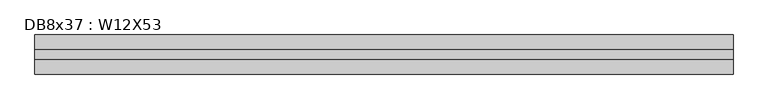
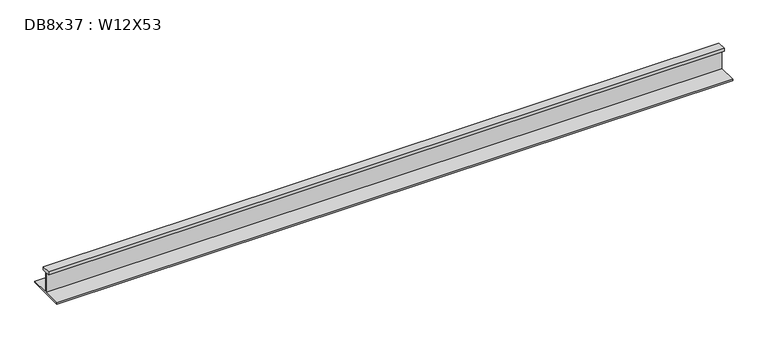
"""IFC4 building model written with IfcOpenShell, lengths in millimetres: beam geometry, DB8x37 : W12X53."""

from ifc_helpers import new_model, si_unit, frame, origin, place, context, project, spatial, polyline, outline, extrude, source, transform, mapped, element, save


def db8x37_w12x53_7e8dff65(model_context):
    return source(origin(), model_context, "Body", "SweptSolid", [
        extrude(outline(polyline([(38.1, 145.415), (38.1, 120.015), (2.921, 120.015), (2.921, -48.4505), (152.4, -48.4505), (152.4, -58.1025), (-152.4, -58.1025), (-152.4, -48.4505), (-2.921, -48.4505), (-2.921, 120.015), (-38.1, 120.015), (-38.1, 145.415), (38.1, 145.415)])), frame((-2793.873, 0.0, 0.0), z_axis=(1.0, 0.0, 0.0), x_axis=(0.0, 1.0, 0.0)), (0.0, 0.0, 1.0), 5438.902),
    ])


if __name__ == "__main__":
    model = new_model("IFC4")
    model_context = context("Model", 3, world=origin())
    ifc_project = project(units=[si_unit("LENGTHUNIT", "METRE", prefix="MILLI")], contexts=[model_context])
    site = spatial("IfcSite", under=ifc_project)
    building = spatial("IfcBuilding", under=site)
    placement = place(None, origin())
    db8x37_w12x53_shape = db8x37_w12x53_7e8dff65(model_context)
    element("IfcBeam", 1, ObjectType="DB8x37 : W12X53", at=placement, inside=building, context=model_context, shape_type="MappedRepresentation", body=[
        mapped(db8x37_w12x53_shape, transform((0.0, 0.0, 0.0), x_axis=(1.0, 0.0, 0.0), y_axis=(0.0, 1.0, 0.0), z_axis=(0.0, 0.0, 1.0))),
    ])
    save(model, "model.ifc")

# Revit data of these elements
# Type "DB8x37 : W12X53"
#   Assembly Code = "B10"
#   W = 53
#   Length [instance default] = 5' - 0"
#   bf = 0' - 10"
#   d = 1' - 0.1"
#   k = 0' - 1 3/8"
#   k2 = 0' - 0.8"
#   tf = 0' - 0.575"
#   tw = 0' - 0.345"
#   A = 0.108333 SF
#   Structural Material [instance default] = Steel ASTM A992
# Element 1 (IfcBeam, "DB8x37 : W12X53")
#   Materials on its faces: "Steel ASTM A992"
# Materials
#   "Steel ASTM A992": class "Metal", colour RGB 199 199 199, transparency 0, Description = "Structural steel 50ksi", Cost = 0
